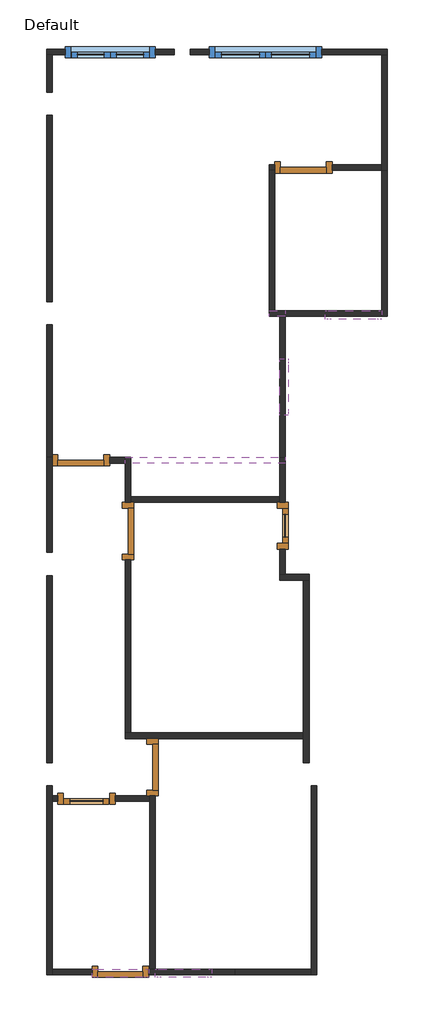
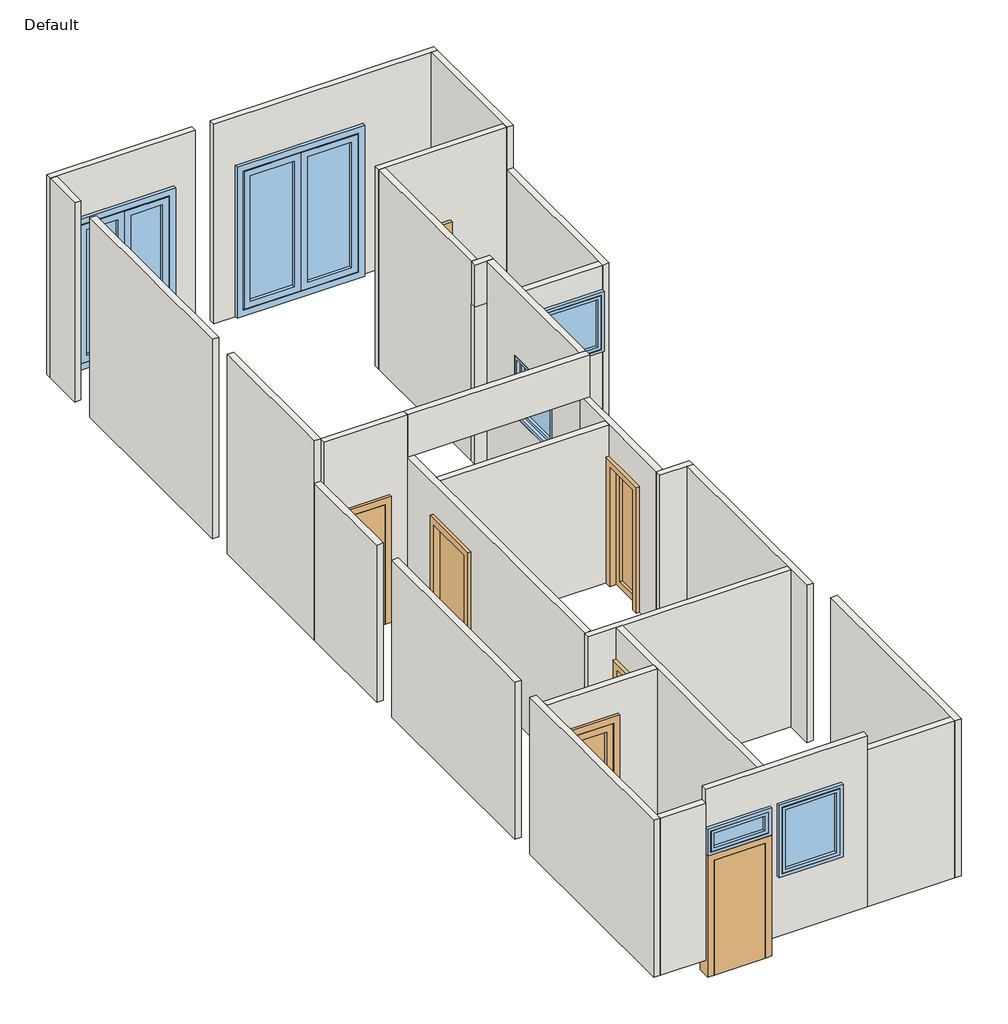
# One storey: 29 walls, 7 doors, 6 windows.
# Revit data of these elements (continued)
# Type "Steel_Wall_3_2 : Steel_Wall_3_2"
#   NameOverride = "Steel_Wall_3_2"
# Type "Steel_Wall_4 : Steel_Wall_4"
#   NameOverride = "Steel_Wall_4"
# Type "Steel_Wall_5 : Steel_Wall_5"
#   NameOverride = "Steel_Wall_5"
# Type "Steel_Wall_6 : Steel_Wall_6"
#   NameOverride = "Steel_Wall_6"
# Type "Steel_Wall_7 : Steel_Wall_7"
#   NameOverride = "Steel_Wall_7"
# Type "Steel_Wall_8_1 : Steel_Wall_8_1"
#   NameOverride = "Steel_Wall_8_1"
# Type "Steel_Wall_8_2 : Steel_Wall_8_2"
#   NameOverride = "Steel_Wall_8_2"
# Type "Steel_Wall_9 : Steel_Wall_9"
#   NameOverride = "Steel_Wall_9"
# Type "Steel_Wall_Bath_1 : Steel_Wall_Bath_1"
#   NameOverride = "Steel_Wall_Bath_1"
# Type "Steel_Wall_Bath_2 : Steel_Wall_Bath_2"
#   NameOverride = "Steel_Wall_Bath_2"
# Type "Steel_Wall_Bath_3 : Steel_Wall_Bath_3"
#   NameOverride = "Steel_Wall_Bath_3"
# Type "Steel_Wall_Bed_1_1 : Steel_Wall_Bed_1_1"
#   NameOverride = "Steel_Wall_Bed_1_1"
# Type "Steel_Wall_Bed_1_2 : Steel_Wall_Bed_1_2"
#   NameOverride = "Steel_Wall_Bed_1_2"
# Type "Steel_Wall_Bed_2_1 : Steel_Wall_Bed_2_1"
#   NameOverride = "Steel_Wall_Bed_2_1"
# Type "Steel_Wall_Bed_2_2 : Steel_Wall_Bed_2_2"
#   NameOverride = "Steel_Wall_Bed_2_2"
# Type "Steel_Wall_Corridor_1 : Steel_Wall_Corridor_1"
#   NameOverride = "Steel_Wall_Corridor_1"
# Type "Steel_Wall_Corridor_2 : Steel_Wall_Corridor_2"
#   NameOverride = "Steel_Wall_Corridor_2"
# Type "Steel_Wall_Kitchen : Steel_Wall_Kitchen"
#   NameOverride = "Steel_Wall_Kitchen"
# Type "Bedroom_1_Window : Bedroom_1_Window"
#   Type Mark = "52"
#   NameOverride = "Bedroom_1_Window"
# Type "Bedroom_1_Window001 : Bedroom_1_Window001"
#   Type Mark = "54"
#   NameOverride = "Bedroom_1_Window001"
# Type "Corridor_Window : Corridor_Window"
#   Type Mark = "55"
#   NameOverride = "Corridor_Window"
# Type "Garden_Door_1 : Garden_Door_1"
#   Type Mark = "50"
#   NameOverride = "Garden_Door_1"
# Type "Garden_Door_2 : Garden_Door_2"
#   Type Mark = "51"
#   NameOverride = "Garden_Door_2"
# Type "Kitchen_Window : Kitchen_Window"
#   Type Mark = "53"
#   NameOverride = "Kitchen_Window"
# Element 1 (IfcDoor, "Bathroom_Door : Bathroom_Door")
#   IfcGUID = "2d9EAMZuD0th02TdqGKw9V"
#   Phase Created = New Construction
#   Materials on its faces: "IfcSurfaceStyle #392"
# Element 2 (IfcDoor, "Bedroom_1_Door : Bedroom_1_Door")
#   IfcGUID = "1_OqppEejAlB8lKkCR4QWC"
#   Phase Created = New Construction
#   Materials on its faces: "IfcSurfaceStyle #392"
# Element 3 (IfcDoor, "Bedroom_2_Door : Bedroom_2_Door")
#   IfcGUID = "2$B6WVKrTAIATxxgFfi0gB"
#   Phase Created = New Construction
#   Materials on its faces: "IfcSurfaceStyle #392"
# Element 4 (IfcDoor, "Bedroom_2__Glass_Door : Bedroom_2__Glass_Door")
#   IfcGUID = "2mkMvagFPD2900nkeEyxCU"
#   Phase Created = New Construction
#   Materials on its faces: "IfcSurfaceStyle #392", "IfcSurfaceStyle #398"
# Element 5 (IfcDoor, "Corridor_Door : Corridor_Door")
#   IfcGUID = "0C86DLcTP6iufxYwWUtltD"
#   Phase Created = New Construction
#   Materials on its faces: "IfcSurfaceStyle #392", "IfcSurfaceStyle #398"
# Element 6 (IfcDoor, "Front_Door : Front_Door")
#   IfcGUID = "3Q78IMAMrFEhyP5s6NcvOq"
#   Phase Created = New Construction
#   Materials on its faces: "IfcSurfaceStyle #392"
# Element 7 (IfcDoor, "Living_Room_Door : Living_Room_Door")
#   IfcGUID = "3k98tirZr53RxQLy$eepBj"
#   Phase Created = New Construction
#   Materials on its faces: "IfcSurfaceStyle #392"
# Element 8 (IfcWall, "Steel_Wall_1 : Steel_Wall_1")
#   IfcGUID = "1kYfjPI1z2dOsmFbZF5vk1"
#   Phase Created = New Construction
#   Materials on its faces: "IfcSurfaceStyle #33"
# Element 9 (IfcWall, "Steel_Wall_10_1 : Steel_Wall_10_1")
#   IfcGUID = "2H1wEzqV97$uYr8_2gY6UW"
#   Phase Created = New Construction
#   Materials on its faces: "IfcSurfaceStyle #33"
# Element 10 (IfcWall, "Steel_Wall_10_2 : Steel_Wall_10_2")
#   IfcGUID = "2KcO0_L111IflKS0Oe9gZ1"
#   Phase Created = New Construction
#   Materials on its faces: "IfcSurfaceStyle #33"
# Element 11 (IfcWall, "Steel_Wall_11 : Steel_Wall_11")
#   IfcGUID = "2lC_UAHmbEbuUifsP1LXZ6"
#   Phase Created = New Construction
#   Materials on its faces: "IfcSurfaceStyle #33"
# Element 12 (IfcWall, "Steel_Wall_12 : Steel_Wall_12")
#   IfcGUID = "2ql$xibhzAeeLpUwcSurNO"
#   Phase Created = New Construction
#   Materials on its faces: "IfcSurfaceStyle #33"
# Element 13 (IfcWall, "Steel_Wall_13 : Steel_Wall_13")
#   IfcGUID = "2Y8TRW6Eb28BE4hqFcYYat"
#   Phase Created = New Construction
#   Materials on its faces: "IfcSurfaceStyle #33"
# Element 14 (IfcWall, "Steel_Wall_14_1 : Steel_Wall_14_1")
#   IfcGUID = "13e6e3AKzBER5jsAP_woOm"
#   Phase Created = New Construction
#   Materials on its faces: "IfcSurfaceStyle #33"
# Element 15 (IfcWall, "Steel_Wall_14_2 : Steel_Wall_14_2")
#   IfcGUID = "2t9TP76RnCBvZR7N7DspqO"
#   Phase Created = New Construction
#   Materials on its faces: "IfcSurfaceStyle #33"
# Element 16 (IfcWall, "Steel_Wall_14_3 : Steel_Wall_14_3")
#   IfcGUID = "3PIBECXaPD8fBrr6oQYvsD"
#   Phase Created = New Construction
#   Materials on its faces: "IfcSurfaceStyle #33"
# Element 17 (IfcWall, "Steel_Wall_2 : Steel_Wall_2")
#   IfcGUID = "28QiRoCobBmQBFVKgJU48$"
#   Phase Created = New Construction
#   Materials on its faces: "IfcSurfaceStyle #33"
# Element 18 (IfcWall, "Steel_Wall_3_1 : Steel_Wall_3_1")
#   IfcGUID = "24zwTt2IT5lPu_PnYAbuQd"
#   Phase Created = New Construction
#   Materials on its faces: "IfcSurfaceStyle #33"
# Element 19 (IfcWall, "Steel_Wall_3_2 : Steel_Wall_3_2")
#   IfcGUID = "1xKmfBGIPAlv3IuhKMrVC6"
#   Phase Created = New Construction
#   Materials on its faces: "IfcSurfaceStyle #33"
# Element 20 (IfcWall, "Steel_Wall_4 : Steel_Wall_4")
#   IfcGUID = "28XGHM95jA2hWOx23ZfQpI"
#   Phase Created = New Construction
#   Materials on its faces: "IfcSurfaceStyle #33"
# Element 21 (IfcWall, "Steel_Wall_5 : Steel_Wall_5")
#   IfcGUID = "2G$YFptgj4Oh0EOEYqEaxI"
#   Phase Created = New Construction
#   Materials on its faces: "IfcSurfaceStyle #33"
# Element 22 (IfcWall, "Steel_Wall_6 : Steel_Wall_6")
#   IfcGUID = "1o9zDiPuLFM9xVI7$R5ryB"
#   Phase Created = New Construction
#   Materials on its faces: "IfcSurfaceStyle #33"
# Element 23 (IfcWall, "Steel_Wall_7 : Steel_Wall_7")
#   IfcGUID = "0$B1TYEDr9MQmvjbWL3brm"
#   Phase Created = New Construction
#   Materials on its faces: "IfcSurfaceStyle #33"
# Element 24 (IfcWall, "Steel_Wall_8_1 : Steel_Wall_8_1")
#   IfcGUID = "0MHnNBBZr1VPIdewH8VvRF"
#   Phase Created = New Construction
#   Materials on its faces: "IfcSurfaceStyle #33"
# Element 25 (IfcWall, "Steel_Wall_8_2 : Steel_Wall_8_2")
#   IfcGUID = "2Cgp0K1rb1Q8_fU3n5VXQo"
#   Phase Created = New Construction
#   Materials on its faces: "IfcSurfaceStyle #33"
# Element 26 (IfcWall, "Steel_Wall_9 : Steel_Wall_9")
#   IfcGUID = "3LPk3dVsL3qRD3WU0CC1fJ"
#   Phase Created = New Construction
#   Materials on its faces: "IfcSurfaceStyle #33"
# Element 27 (IfcWall, "Steel_Wall_Bath_1 : Steel_Wall_Bath_1")
#   IfcGUID = "1q1P9RGs56xRJsdUQ4c$iv"
#   Phase Created = New Construction
#   Materials on its faces: "IfcSurfaceStyle #33"
# Element 28 (IfcWall, "Steel_Wall_Bath_2 : Steel_Wall_Bath_2")
#   IfcGUID = "0bB8O9Uzr7W9xbZH93qA5G"
#   Phase Created = New Construction
#   Materials on its faces: "IfcSurfaceStyle #33"
# Element 29 (IfcWall, "Steel_Wall_Bath_3 : Steel_Wall_Bath_3")
#   IfcGUID = "1yRRlDjj1AH8szfMVlF9gK"
#   Phase Created = New Construction
#   Materials on its faces: "IfcSurfaceStyle #33"
# Element 30 (IfcWall, "Steel_Wall_Bed_1_1 : Steel_Wall_Bed_1_1")
#   IfcGUID = "0fsryBmy92HxbeEe0VAP5z"
#   Phase Created = New Construction
#   Materials on its faces: "IfcSurfaceStyle #33"
# Element 31 (IfcWall, "Steel_Wall_Bed_1_2 : Steel_Wall_Bed_1_2")
#   IfcGUID = "3IqxH_DyHDtP$IUvlhbDBV"
#   Phase Created = New Construction
#   Materials on its faces: "IfcSurfaceStyle #33"
# Element 32 (IfcWall, "Steel_Wall_Bed_2_1 : Steel_Wall_Bed_2_1")
#   IfcGUID = "2FEIiMdgXB5hxET7ecChMF"
#   Phase Created = New Construction
#   Materials on its faces: "IfcSurfaceStyle #33"
# Element 33 (IfcWall, "Steel_Wall_Bed_2_2 : Steel_Wall_Bed_2_2")
#   IfcGUID = "2XSrZAOpP9ygM8yaoyXRZv"
#   Phase Created = New Construction
#   Materials on its faces: "IfcSurfaceStyle #33"
# Element 34 (IfcWall, "Steel_Wall_Corridor_1 : Steel_Wall_Corridor_1")
#   IfcGUID = "2WpmdWzI12XAh4Cz3rhidj"
#   Phase Created = New Construction
#   Materials on its faces: "IfcSurfaceStyle #33"
# Element 35 (IfcWall, "Steel_Wall_Corridor_2 : Steel_Wall_Corridor_2")
#   IfcGUID = "1LowZ9Ljz0uu9eh$WESGHl"
#   Phase Created = New Construction
#   Materials on its faces: "IfcSurfaceStyle #33"
# Element 36 (IfcWall, "Steel_Wall_Kitchen : Steel_Wall_Kitchen")
#   IfcGUID = "25Aek3czj16xSehWca_NKz"
#   Phase Created = New Construction
#   Materials on its faces: "IfcSurfaceStyle #33"
# Element 37 (IfcWindow, "Bedroom_1_Window : Bedroom_1_Window")
#   IfcGUID = "3fbRgI4x53buaM79E0m8n$"
#   Mark = "6"
#   Phase Created = New Construction
#   Materials on its faces: "IfcSurfaceStyle #392", "IfcSurfaceStyle #398"
# Element 38 (IfcWindow, "Bedroom_1_Window001 : Bedroom_1_Window001")
#   IfcGUID = "1_eskcO1D8ewmErJWrP0qK"
#   Mark = "10"
#   Phase Created = New Construction
#   Materials on its faces: "IfcSurfaceStyle #392", "IfcSurfaceStyle #398"
# Element 39 (IfcWindow, "Corridor_Window : Corridor_Window")
#   IfcGUID = "16kYNChfDBAgUE7heRcWn$"
#   Mark = "12"
#   Phase Created = New Construction
#   Materials on its faces: "IfcSurfaceStyle #392", "IfcSurfaceStyle #398"
# Element 40 (IfcWindow, "Garden_Door_1 : Garden_Door_1")
#   IfcGUID = "14Z0K45SrC3OmOkzA2_FH1"
#   Mark = "2"
#   Phase Created = New Construction
#   Materials on its faces: "IfcSurfaceStyle #392", "IfcSurfaceStyle #398"
# Element 41 (IfcWindow, "Garden_Door_2 : Garden_Door_2")
#   IfcGUID = "3wrQCLCwbEtwn8FcH1Y$Y3"
#   Mark = "4"
#   Phase Created = New Construction
#   Materials on its faces: "IfcSurfaceStyle #392", "IfcSurfaceStyle #398"
# Element 42 (IfcWindow, "Kitchen_Window : Kitchen_Window")
#   IfcGUID = "1EPiASaIX6Kurp1E7ijjMw"
#   Mark = "8"
#   Phase Created = New Construction
#   Materials on its faces: "IfcSurfaceStyle #392", "IfcSurfaceStyle #398"
# Materials
#   "IfcSurfaceStyle #392": class "Unassigned", colour RGB 204 204 204, transparency 0
#   "IfcSurfaceStyle #398": class "Unassigned", colour RGB 93 183 203, transparency 0.85
#   "IfcSurfaceStyle #33": class "Unassigned", colour RGB 214 214 214, transparency 0
